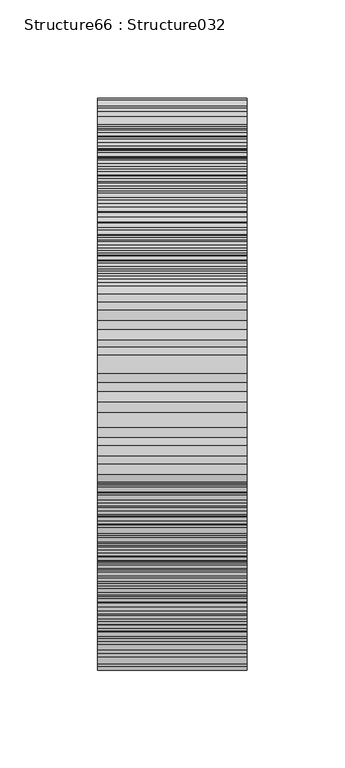
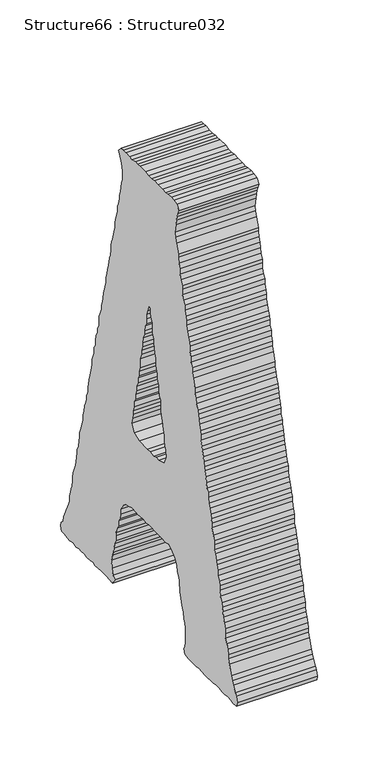
"""IFC4 building model written with IfcOpenShell, lengths in millimetres: proxy geometry, Structure66 : Structure032."""

from ifc_helpers import new_model, si_unit, frame, origin, place, context, project, spatial, polyline, outline, extrude, source, transform, mapped, element, save


def structure66_structure032_756e5080(model_context):
    return source(origin(), model_context, "Body", "SweptSolid", [
        extrude(outline(polyline([(275009.5661122, 3818.8310229), (275009.5661122, 3814.7296538), (275010.7262412, 3811.2043377), (275013.0657546, 3805.9476534), (275013.0657546, 3801.8462843), (275013.6450168, 3795.960595), (275016.0069946, 3791.8865042), (275016.0069946, 3787.7867397), (275018.3481126, 3783.0868532), (275018.9498392, 3777.8285642), (275018.9498392, 3773.11905), (275021.2668881, 3769.6274306), (275021.2668881, 3763.759392), (275023.0271393, 3759.6596275), (275024.788995, 3755.559863), (275024.788995, 3750.8583719), (275025.9699839, 3746.1745313), (275028.2870328, 3737.400554), (275029.4680217, 3732.1149867), (275030.6490106, 3727.4311462), (275031.8299995, 3723.3313817), (275031.8299995, 3718.6571688), (275033.5918553, 3713.3555556), (275034.1711175, 3709.2718371), (275035.9089042, 3704.5879966), (275037.0898931, 3701.0723082), (275037.6691553, 3695.786741), (275039.431011, 3690.512406), (275039.431011, 3685.8285655), (275040.6119999, 3682.8857208), (275041.7929888, 3677.6274319), (275043.5307755, 3672.9435914), (275045.2910266, 3668.8261762), (275045.8702889, 3664.1423357), (275046.4720156, 3660.0682449), (275047.0528824, 3654.1841602), (275049.4148602, 3650.1004418), (275049.9941224, 3645.9830266), (275050.5509202, 3641.2991861), (275051.1526469, 3636.0408972), (275052.3336358, 3631.915459), (275054.0938869, 3627.8397636), (275055.8557426, 3622.555801), (275057.0142671, 3617.2718384), (275057.0142671, 3613.772196), (275057.6159938, 3607.8961343), (275059.3537804, 3604.3964919), (275060.5347694, 3600.2967274), (275061.6948984, 3595.5872132), (275062.2966251, 3589.7544759), (275063.477614, 3586.2115092), (275067.554914, 3577.4535778), (275069.9184964, 3572.1423369), (275071.6787476, 3568.6426945), (275072.8148076, 3563.366755), (275075.7560476, 3560.441561), (275076.9386411, 3556.3417965), (275075.1767854, 3551.6675836), (275070.4977587, 3551.6675836), (275065.7946629, 3551.0658569), (275061.6948984, 3550.4833855), (275056.4350049, 3551.6675836), (275051.1526469, 3550.4833855), (275046.4720156, 3551.6675836), (275042.9515133, 3551.0658569), (275037.0898931, 3551.6675836), (275033.5918553, 3551.0658569), (275027.7077706, 3551.0658569), (275023.6064015, 3551.6675836), (275019.5291015, 3551.0658569), (275014.8260057, 3551.0658569), (275010.146979, 3551.6675836), (275000.7632519, 3551.6675836), (274996.0842252, 3551.0658569), (274990.8018672, 3550.4833855), (274987.3022248, 3556.3417965), (274990.222605, 3559.2669905), (274991.9828561, 3565.1254015), (274992.5621183, 3572.7440636), (274990.8018672, 3578.6104977), (274989.0640805, 3582.7102621), (274988.4623538, 3587.3860796), (274987.8830916, 3592.0955938), (274985.5195092, 3596.7698067), (274985.5195092, 3601.4536473), (274984.940247, 3604.9709403), (274983.759258, 3610.2292293), (274981.4422092, 3613.772196), (274980.8629469, 3619.6145609), (274979.0786267, 3622.555801), (274977.9201023, 3627.8397636), (274977.9201023, 3633.0980525), (274973.2410756, 3639.5405396), (274969.7189687, 3643.0578326), (274962.6763596, 3644.8245022), (274959.1783218, 3645.9830266), (274953.2942371, 3645.4262289), (274949.2153325, 3644.8245022), (274944.5363058, 3645.4262289), (274939.83321, 3645.9830266), (274935.7334455, 3644.8245022), (274930.4510875, 3645.4262289), (274918.1485848, 3645.4262289), (274912.2869646, 3644.8245022), (274902.9048421, 3644.8245022), (274898.2258154, 3645.9830266), (274891.784933, 3642.4833842), (274887.6835639, 3638.9580681), (274884.7647883, 3633.0980525), (274883.5837994, 3627.2396415), (274881.8219436, 3622.555801), (274880.6409547, 3619.6145609), (274879.4824303, 3609.0723094), (274878.3014414, 3604.3964919), (274877.1429169, 3600.2967274), (274875.3810612, 3596.1953583), (274874.2000723, 3592.0955938), (274873.6208101, 3586.2115092), (274871.8605589, 3582.7102621), (274870.67957, 3578.6104977), (274870.67957, 3573.9266571), (274870.67957, 3563.9412034), (274871.8605589, 3559.2669905), (274873.6208101, 3555.7416744), (274871.2812967, 3551.6675836), (274865.9989387, 3550.4833855), (274852.5379116, 3550.4833855), (274848.4156827, 3551.6675836), (274843.1557891, 3551.0658569), (274838.4751578, 3550.4833855), (274834.3529289, 3550.4833855), (274828.5137731, 3551.0658569), (274824.4140086, 3551.0658569), (274819.7109128, 3551.6675836), (274815.6095437, 3551.6675836), (274810.930517, 3550.4833855), (274805.648159, 3550.4833855), (274800.9675277, 3551.6675836), (274795.6867743, 3551.0658569), (274792.1871319, 3550.4833855), (274786.3255117, 3551.0658569), (274785.1445228, 3555.1848766), (274786.9063785, 3560.441561), (274788.064903, 3563.366755), (274791.5854052, 3568.6426945), (274793.3456564, 3572.1423369), (274795.1299766, 3576.2693797), (274798.0262877, 3586.2115092), (274799.7865388, 3590.3289243), (274799.7865388, 3594.4286888), (274800.9675277, 3599.1125293), (274802.1501212, 3604.3964919), (274804.4671701, 3608.4705827), (274805.0688968, 3612.5976255), (274805.0688968, 3617.2718384), (274806.2498857, 3622.555801), (274808.0101368, 3627.2396415), (274808.5893991, 3632.5155811), (274809.7719926, 3636.0408972), (274810.930517, 3640.114988), (274812.6907682, 3645.4262289), (274813.8492926, 3650.6845178), (274813.8492926, 3655.3587307), (274815.0302815, 3659.4584952), (274817.3938639, 3663.5598643), (274817.3938639, 3668.8261762), (274819.1316506, 3673.5276674), (274819.7109128, 3677.0449605), (274821.471164, 3682.8857208), (274822.6521529, 3686.4030139), (274822.6521529, 3691.0868544), (274823.2314151, 3695.2122926), (274824.4140086, 3699.8881101), (274826.7310575, 3705.7545441), (274826.7310575, 3710.4560353), (274827.9120464, 3714.5301261), (274829.0930353, 3718.0554422), (274830.2740242, 3723.3313817), (274832.03588, 3727.4311462), (274833.1944044, 3732.7167134), (274833.1944044, 3737.9750024), (274834.9546555, 3740.9162424), (274836.11318, 3745.6000829), (274836.7149067, 3751.4424479), (274838.4751578, 3756.1423345), (274839.6577513, 3759.6596275), (274840.2370135, 3764.3611187), (274840.7938113, 3769.0176809), (274842.5540624, 3774.3032481), (274843.1557891, 3777.8285642), (274844.9160402, 3783.0868532), (274844.9160402, 3788.3611881), (274846.0970292, 3791.8865042), (274847.8364204, 3797.1463977), (274848.4156827, 3801.8462843), (274849.5966716, 3806.5317294), (274850.1759338, 3810.0474179), (274852.5379116, 3815.3313805), (274853.6980407, 3820.015221), (274854.8790296, 3824.1149855), (274854.8790296, 3829.374879), (274857.7978051, 3837.6000817), (274858.978794, 3842.8583706), (274859.5580563, 3846.9757858), (274861.319912, 3851.6612309), (274861.319912, 3856.9179152), (274863.0576987, 3861.0192843), (274863.6594254, 3866.3032469), (274864.2386876, 3869.8189354), (274865.9989387, 3873.9203044), (274867.7591898, 3878.5784713), (274868.9417834, 3883.8881076), (274868.9417834, 3888.5623205), (274870.1227723, 3892.6636896), (274871.8605589, 3897.3475301), (274871.8605589, 3902.6314927), (274874.2000723, 3906.1487857), (274875.3810612, 3910.8310217), (274875.961928, 3916.0909152), (274875.961928, 3919.6066036), (274878.3014414, 3924.2888396), (274879.4824303, 3928.9919353), (274880.0616925, 3934.2758979), (274881.2426814, 3938.9517154), (274882.4236703, 3944.235678), (274882.4236703, 3947.1496398), (274885.9233127, 3956.5349715), (274887.0818372, 3961.794865), (274888.2628261, 3965.8930249), (274886.502575, 3974.7055128), (274885.3215861, 3979.9621971), (274884.7647883, 3983.4794902), (274883.5837994, 3987.5792547), (274881.2426814, 3991.6806238), (274884.7647883, 3996.390138), (274890.0230772, 3996.9645864), (274894.1244463, 3997.5486624), (274899.4068043, 3997.5486624), (274903.5065688, 3996.390138), (274908.7664623, 3996.9645864), (274916.3883337, 3996.9645864), (274921.6706917, 3997.5486624), (274926.9514451, 3996.390138), (274931.6320764, 3996.390138), (274936.3127077, 3997.5486624), (274945.6723657, 3997.5486624), (274949.7945947, 3996.9645864), (274953.2942371, 3997.5486624), (274958.5765951, 3996.390138), (274963.2556218, 3996.390138), (274968.5379798, 3997.5486624), (274972.6393489, 3997.5486624), (274976.7391134, 3996.9645864), (274980.8629469, 3992.2614906), (274978.4993645, 3987.5792547), (274976.7391134, 3984.0635662), (274975.5581245, 3979.3781211), (274974.3996, 3974.7055128), (274974.3996, 3966.5043792), (274976.1598512, 3962.3757319), (274977.3183756, 3957.1190475), (274977.9201023, 3952.435207), (274979.6803534, 3947.7337158), (274979.6803534, 3944.235678), (274980.8629469, 3938.3499888), (274982.6231981, 3934.8503464), (274982.6231981, 3929.5904528), (274984.3609847, 3924.8905662), (274986.1212359, 3919.6066036), (274987.3022248, 3915.5068392), (274987.3022248, 3910.8310217), (274988.4623538, 3906.1487857), (274989.6433427, 3902.6314927), (274990.8018672, 3896.763454), (274992.5621183, 3893.822214), (274993.7431072, 3888.5623205), (274993.7431072, 3884.4609514), (274994.3223694, 3878.5784713), (274996.0842252, 3875.0772243), (274996.6634874, 3870.4030114), (274997.8220118, 3866.3032469), (274999.0030008, 3861.0192843), (275000.1839897, 3856.9179152), (275001.9442408, 3851.6612309), (275001.9442408, 3846.9757858), (275003.7060965, 3841.6741725), (275004.2853588, 3838.1761347), (275006.0231454, 3833.4730389), (275006.6248721, 3828.2163546), (275007.2041343, 3824.1149855), (275009.5661122, 3818.8310229)]), holes=[polyline([(274946.8533546, 3720.4158154), (274955.0544882, 3723.9154578), (274958.5765951, 3730.9323932), (274957.416466, 3736.7988273), (274956.2354771, 3741.5003184), (274956.2354771, 3744.9999608), (274954.475226, 3750.3015741), (274954.475226, 3755.559863), (274952.7149749, 3759.0595054), (274952.1357126, 3764.3611187), (274950.9771882, 3768.4432325), (274950.9771882, 3773.11905), (274948.6136058, 3777.8285642), (274948.6136058, 3783.0868532), (274946.8533546, 3786.0280932), (274946.2740924, 3790.7039107), (274945.115568, 3795.4037973), (274944.5363058, 3804.7730829), (274942.77445, 3810.0474179), (274942.1727233, 3814.7296538), (274940.9917344, 3818.8310229), (274940.4124722, 3822.932392), (274939.83321, 3828.790803), (274937.4936966, 3833.4730389), (274937.4936966, 3836.9919366), (274936.9144344, 3842.2758992), (274934.550852, 3845.8012153), (274934.550852, 3851.0595042), (274933.9715898, 3855.7353217), (274932.2113386, 3860.4432313), (274931.0303497, 3865.1190488), (274929.292563, 3864.5446004), (274929.292563, 3860.4432313), (274928.1115741, 3856.3161885), (274926.3497184, 3851.6612309), (274926.3497184, 3846.3772683), (274925.7704562, 3842.2758992), (274923.4084784, 3837.6000817), (274923.4084784, 3832.8921721), (274922.8292161, 3828.790803), (274921.6706917, 3824.1149855), (274920.5105626, 3819.4150989), (274919.908836, 3813.5743386), (274919.3295737, 3810.0474179), (274917.5693226, 3805.9476534), (274917.5693226, 3800.6717138), (274915.2298092, 3795.4037973), (274915.2298092, 3790.7039107), (274914.0488203, 3786.0280932), (274912.2869646, 3782.5027771), (274911.7077024, 3777.2444882), (274911.7077024, 3772.5606477), (274911.1284402, 3767.8607611), (274909.368189, 3763.759392), (274908.7664623, 3759.6596275), (274908.1872001, 3754.9854146), (274905.8476868, 3750.8583719), (274906.4494134, 3744.9999608), (274905.2668199, 3740.9162424), (274904.085831, 3736.7988273), (274902.9048421, 3730.9323932), (274905.8476868, 3723.3313817), (274914.650547, 3720.4158154), (274918.727847, 3720.9726131), (274922.8292161, 3719.8140887), (274928.1115741, 3720.9726131), (274933.3923275, 3720.4158154), (274946.8533546, 3720.4158154)])]), frame((-59031.6926606, 0.0, 0.0), z_axis=(1.0, 0.0, 0.0), x_axis=(0.0, 1.0, 0.0)), (0.0, 0.0, 1.0), 76.2),
    ])


if __name__ == "__main__":
    model = new_model("IFC4")
    model_context = context("Model", 3, world=origin())
    ifc_project = project(units=[si_unit("LENGTHUNIT", "METRE", prefix="MILLI")], contexts=[model_context])
    site = spatial("IfcSite", under=ifc_project)
    building = spatial("IfcBuilding", under=site)
    placement = place(None, origin())
    structure66_structure032_shape = structure66_structure032_756e5080(model_context)
    element("IfcBuildingElementProxy", 1, Name="Structure66 : Structure032", ObjectType="Structure66 : Structure032", at=placement, inside=building, context=model_context, shape_type="MappedRepresentation", body=[
        mapped(structure66_structure032_shape, transform((0.0, 0.0, 0.0), x_axis=(1.0, 0.0, 0.0), y_axis=(0.0, 1.0, 0.0), z_axis=(0.0, 0.0, 1.0))),
    ])
    save(model, "model.ifc")

# Revit data of these elements
# Type "Structure66 : Structure032"
#   NameOverride = "Structure032"
# Element 1 (IfcBuildingElementProxy, "Structure66 : Structure032")
#   Materials on its faces: "BRUSHED ALUM. LETTERING"
# Materials
#   "BRUSHED ALUM. LETTERING": class "Unassigned", colour RGB 169 181 186, transparency 0, Cost = 0
